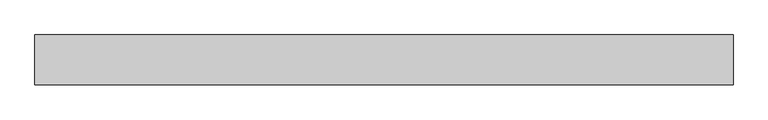
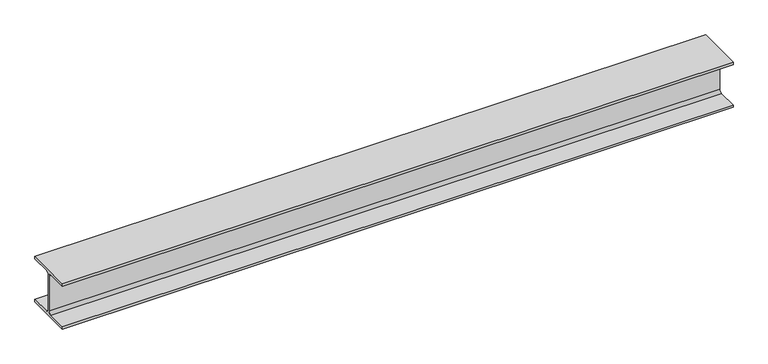
"""IFC4 building model written with IfcOpenShell, lengths in millimetres: beam geometry, 0912_Steel Framing_H-KSD3502 : H_SB_ASB_H-300x300x10x15."""

from ifc_helpers import new_model, si_unit, point, frame, frame_2d, origin, place, context, project, spatial, polyline, circle_curve, trimmed, segment, composite_curve, outline, extrude, source, transform, mapped, element, save


def beam_bb6acfee(model_context):
    return source(origin(), model_context, "Body", "SweptSolid", [
        extrude(outline(composite_curve([segment(polyline([(150.0, -135.0), (150.0, -150.0), (-150.0, -150.0), (-150.0, -135.0), (-23.0, -135.0)]), True, "CONTINUOUS"), segment(trimmed(circle_curve(frame_2d((-23.0, -117.0)), 18.0), [point((-23.0, -135.0))], [point((-5.0, -117.0))], True, "CARTESIAN"), True, "CONTINUOUS"), segment(polyline([(-5.0, -117.0), (-5.0, 117.0)]), True, "CONTINUOUS"), segment(trimmed(circle_curve(frame_2d((-23.0, 117.0)), 18.0), [point((-5.0, 117.0))], [point((-23.0, 135.0))], True, "CARTESIAN"), True, "CONTINUOUS"), segment(polyline([(-23.0, 135.0), (-150.0, 135.0), (-150.0, 150.0), (150.0, 150.0), (150.0, 135.0), (23.0, 135.0)]), True, "CONTINUOUS"), segment(trimmed(circle_curve(frame_2d((23.0, 117.0)), 18.0), [point((23.0, 135.0))], [point((5.0, 117.0))], True, "CARTESIAN"), True, "CONTINUOUS"), segment(polyline([(5.0, 117.0), (5.0, -117.0)]), True, "CONTINUOUS"), segment(trimmed(circle_curve(frame_2d((23.0, -117.0)), 18.0), [point((5.0, -117.0))], [point((23.0, -135.0))], True, "CARTESIAN"), True, "CONTINUOUS"), segment(polyline([(23.0, -135.0), (150.0, -135.0)]), True, "CONTINUOUS")], self_intersect=False)), frame((-2849.2330406, 0.0, 0.0), z_axis=(1.0, 0.0, 0.0), x_axis=(0.0, 1.0, 0.0)), (0.0, 0.0, 1.0), 4213.4660812),
    ])


if __name__ == "__main__":
    model = new_model("IFC4")
    model_context = context("Model", 3, world=origin())
    ifc_project = project(units=[si_unit("LENGTHUNIT", "METRE", prefix="MILLI")], contexts=[model_context])
    site = spatial("IfcSite", under=ifc_project)
    building = spatial("IfcBuilding", under=site)
    placement = place(None, origin())
    beam_shape = beam_bb6acfee(model_context)
    element("IfcBeam", 1, ObjectType="0912_Steel Framing_H-KSD3502 : H_SB_ASB_H-300x300x10x15", at=placement, inside=building, context=model_context, shape_type="MappedRepresentation", body=[
        mapped(beam_shape, transform((0.0, 0.0, 0.0), x_axis=(1.0, 0.0, 0.0), y_axis=(0.0, 1.0, 0.0), z_axis=(0.0, 0.0, 1.0))),
    ])
    save(model, "model.ifc")

# Revit data of these elements
# Type "0912_Steel Framing_H-KSD3502 : H_SB_ASB_H-300x300x10x15"
#   H_WM Code_1 = "S01AA001-00001 | Main Steel Structure Fabrication Work | Shelter/Building | Heavy Steel - Standard (Weight≥90KG/M) | Material: (   )"
#   H_WM Code_2 = "S03AA027-00001 | Main Steel Structure Erection Work | Shelter/Building | Heavy Steel (Weight≥90KG/M) | Material: (   )"
#   H_WM Code_3 = "S01AA010-00001 | Main Steel Structure Fabrication Work | Shelter/Building | Steel Painting/Coating | for Non-Fireproofed Steel Surface, Surface Preparation, Primer, Second & Final Coat | Material: (   )"
#   H_Q'ty Cal Type Tag = "SB-Q2"
#   Width = 30.0 cm
#   Web Thickness = 1.0 cm
#   Web Fillet = 1.8 cm
#   Warping Constant = 1370000.0 cm⁶
#   W = 0
#   Torsional Moment of Inertia = 77.00 cm⁴
#   Section Area = 119.8 cm²
#   Plastic Modulus weak axis = 684.0 cm³
#   Plastic Modulus strong axis = 1500.0 cm³
#   Perimeter = 1.75 m²/m
#   Nominal Weight = 94.00 kgf/m
#   Moment of Inertia weak axis = 6750.00 cm⁴
#   Moment of Inertia strong axis = 20400.00 cm⁴
#   Height = 30.0 cm
#   Flange Thickness = 1.5 cm
#   Elastic Modulus weak axis = 450.0 cm³
#   Elastic Modulus strong axis = 1360.0 cm³
#   Centroid Vertical = 15.0 cm
#   Centroid Horizontal = 15.0 cm
#   Ix = 204000000
#   Length [instance default] = 1.5240 m
#   Zx = 1500000
#   b = 0.3000 m
#   h = 0.3000 m
#   r = 0.0180 m
#   s = 0.0100 m
#   t = 0.0150 m
#   A = 0.01198 m²
#   Structural Material [instance default] = Steel, 45-345
#   Assembly Code = ""
# Element 1 (IfcBeam, "0912_Steel Framing_H-KSD3502 : H_SB_ASB_H-300x300x10x15")
#   Structural Material = none
# Materials
#   "Steel, 45-345": class "Metal", colour RGB 189 187 185, transparency 0, Description = "Steel 345 MPa", Cost = 0
